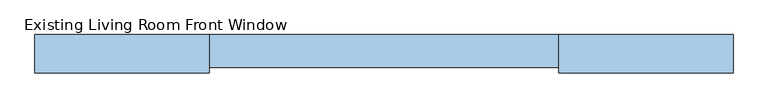
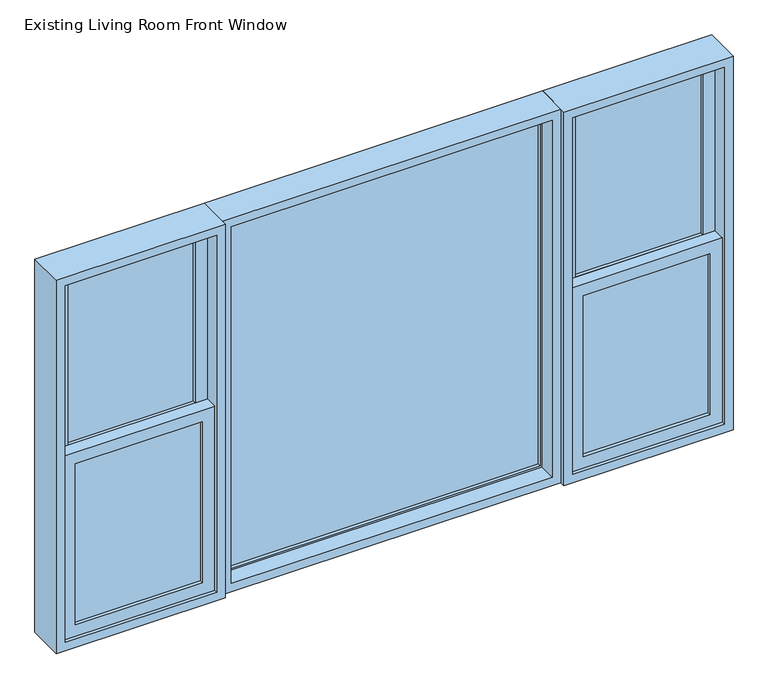
"""IFC4 building model written with IfcOpenShell, lengths in millimetres: window geometry, Existing Living Room Front Window."""

import ifcopenshell
import ifcopenshell.guid

model = None  # the IFC model being written
_history = None  # IfcOwnerHistory: only IFC2X3 demands one
_inside = {}  # id of a spatial element -> (the spatial element, [elements in it])
_under = {}  # id of a project, library or spatial element -> (it, [spatial elements below it])
_declared = {}  # id of a project -> (the project, [libraries it declares])
_typed = {}  # id of a type object -> (the type object, [elements of that type])
_made_of = {}  # id of a material, layer set ... -> (it, [elements and type objects made of it])


def new_model(schema):
    """Start an empty IFC model of exactly this schema.

    Asked for "IFC4X3", IfcOpenShell would pick the latest addendum, in which some entities
    have other attributes; the version numbers below select the first issue.
    IFC2X3 requires an IfcOwnerHistory on every rooted entity: one is made here for all.
    """
    global model, _history
    if schema == "IFC4X3":
        model = ifcopenshell.file(schema_version=(4, 3, 0, 0))
    else:
        model = ifcopenshell.file(schema=schema)
    _inside.clear()
    _under.clear()
    _declared.clear()
    _typed.clear()
    _made_of.clear()
    _history = None
    if model.schema == "IFC2X3":
        org = make("IfcOrganization", Name="unknown")
        user = make(
            "IfcPersonAndOrganization",
            ThePerson=make("IfcPerson", FamilyName="unknown"),
            TheOrganization=org,
        )
        app = make(
            "IfcApplication",
            ApplicationDeveloper=org,
            Version="unknown",
            ApplicationFullName="unknown",
            ApplicationIdentifier="unknown",
        )
        _history = make(
            "IfcOwnerHistory",
            OwningUser=user,
            OwningApplication=app,
            ChangeAction="ADDED",
            CreationDate=0,
        )
    return model


def make(cls, **values):
    """One entity of the class cls with the attributes given. An attribute that is None is left unset."""
    return model.create_entity(
        cls, **{name: value for name, value in values.items() if value is not None}
    )


def rooted(cls, **values):
    """An entity with a GlobalId (a new one), such as an element, a storey or a relation."""
    return make(cls, GlobalId=ifcopenshell.guid.new(), OwnerHistory=_history, **values)


def si_unit(unit_type, name, prefix=None):
    """IfcSIUnit, for example si_unit("LENGTHUNIT", "METRE", prefix="MILLI")."""
    return make("IfcSIUnit", UnitType=unit_type, Prefix=prefix, Name=name)


def assignment(units):
    """IfcUnitAssignment: the units of a project."""
    return None if units is None else make("IfcUnitAssignment", Units=units)


def point(xyz):
    """IfcCartesianPoint."""
    return None if xyz is None else make("IfcCartesianPoint", Coordinates=xyz)


def direction(xyz):
    """IfcDirection."""
    return None if xyz is None else make("IfcDirection", DirectionRatios=xyz)


def frame(location, z_axis=None, x_axis=None):
    """IfcAxis2Placement3D, a coordinate frame: its origin and axes. An axis left out is left unset."""
    return make(
        "IfcAxis2Placement3D",
        Location=point(location),
        Axis=direction(z_axis),
        RefDirection=direction(x_axis),
    )


def origin():
    """The frame at (0, 0, 0) with its axes left unset."""
    return frame((0.0, 0.0, 0.0))


def place(relative_to, where):
    """IfcLocalPlacement: puts the frame where relative to a parent placement (None: the world)."""
    return make(
        "IfcLocalPlacement", PlacementRelTo=relative_to, RelativePlacement=where
    )


def context(
    kind, dimensions, precision=None, world=None, true_north=None, identifier=None
):
    """IfcGeometricRepresentationContext, for example the 3D "Model" context."""
    return make(
        "IfcGeometricRepresentationContext",
        ContextIdentifier=identifier,
        ContextType=kind,
        CoordinateSpaceDimension=dimensions,
        Precision=precision,
        WorldCoordinateSystem=world,
        TrueNorth=true_north,
    )


def project(units=None, contexts=None):
    """IfcProject with its units and contexts."""
    return rooted(
        "IfcProject",
        Name="project",
        RepresentationContexts=contexts,
        UnitsInContext=assignment(units),
    )


def spatial(cls, under=None, at=None, **own):
    """A site, building, storey or space (cls), placed at a placement, below another one or the project."""
    s = rooted(cls, ObjectPlacement=at, **own)
    if under is not None:
        _under.setdefault(under.id(), (under, []))[1].append(s)
    return s


def polyline(points):
    """IfcPolyline through the points."""
    return make("IfcPolyline", Points=[point(p) for p in points])


def outline(outer, holes=None, kind="AREA"):
    """IfcArbitraryClosedProfileDef: a profile drawn as a closed curve; with holes, ...WithVoids."""
    if holes is None:
        return make("IfcArbitraryClosedProfileDef", ProfileType=kind, OuterCurve=outer)
    return make(
        "IfcArbitraryProfileDefWithVoids",
        ProfileType=kind,
        OuterCurve=outer,
        InnerCurves=holes,
    )


def extrude(swept, where, along, depth):
    """IfcExtrudedAreaSolid: the profile swept, set in the frame where, extruded along a direction by depth."""
    return make(
        "IfcExtrudedAreaSolid",
        SweptArea=swept,
        Position=where,
        ExtrudedDirection=direction(along),
        Depth=depth,
    )


def faces_of(points, faces, orient=None, outer=None):
    """IfcFace entities. A face is a list of loops; a loop is a list of indices into points, from 0.

    orient and outer hold one flag for each loop. By default every Orientation is true, the
    first loop of a face is its IfcFaceOuterBound and the others are IfcFaceBound.
    """
    made = []
    for i, loops in enumerate(faces):
        bounds = []
        for j, loop in enumerate(loops):
            is_outer = j == 0 if outer is None else outer[i][j]
            bounds.append(
                make(
                    "IfcFaceOuterBound" if is_outer else "IfcFaceBound",
                    Bound=make("IfcPolyLoop", Polygon=[points[k] for k in loop]),
                    Orientation=True if orient is None else orient[i][j],
                )
            )
        made.append(make("IfcFace", Bounds=bounds))
    return made


def faceted_brep(points, faces, orient=None, outer=None, voids=None):
    """IfcFacetedBrep: a solid bounded by flat faces; with voids (closed shells), ...WithVoids."""
    shared = [point(p) for p in points]
    hull = make("IfcClosedShell", CfsFaces=faces_of(shared, faces, orient, outer))
    if voids is None:
        return make("IfcFacetedBrep", Outer=hull)
    return make(
        "IfcFacetedBrepWithVoids",
        Outer=hull,
        Voids=[
            make(cls, CfsFaces=faces_of(shared, fs, o, b)) for cls, fs, o, b in voids
        ],
    )


def shape(context_of_items, identifier, shape_type, items):
    """IfcShapeRepresentation: the items that make up one representation, for example the "Body"."""
    return make(
        "IfcShapeRepresentation",
        ContextOfItems=context_of_items,
        RepresentationIdentifier=identifier,
        RepresentationType=shape_type,
        Items=items,
    )


def source(mapping_origin, context_of_items, identifier, shape_type, items):
    """IfcRepresentationMap: a shape defined once, which mapped items show again and again."""
    return make(
        "IfcRepresentationMap",
        MappingOrigin=mapping_origin,
        MappedRepresentation=shape(context_of_items, identifier, shape_type, items),
    )


def transform(
    local_origin,
    x_axis=None,
    y_axis=None,
    z_axis=None,
    scale=None,
    scale2=None,
    scale3=None,
    uniform=True,
):
    """IfcCartesianTransformationOperator3D, or its non-uniform kind. x_axis, y_axis, z_axis: its Axis1, 2, 3."""
    if uniform:
        return make(
            "IfcCartesianTransformationOperator3D",
            Axis1=direction(x_axis),
            Axis2=direction(y_axis),
            LocalOrigin=point(local_origin),
            Scale=scale,
            Axis3=direction(z_axis),
        )
    return make(
        "IfcCartesianTransformationOperator3DnonUniform",
        Axis1=direction(x_axis),
        Axis2=direction(y_axis),
        LocalOrigin=point(local_origin),
        Scale=scale,
        Axis3=direction(z_axis),
        Scale2=scale2,
        Scale3=scale3,
    )


def mapped(mapping_source, mapping_target):
    """IfcMappedItem: shows the shape of a source again, moved by a transform."""
    return make(
        "IfcMappedItem", MappingSource=mapping_source, MappingTarget=mapping_target
    )


def made_of(thing, what):
    """Note that an element or type object is made of a material, layer set ...; save() writes the relation."""
    if what is not None:
        _made_of.setdefault(what.id(), (what, []))[1].append(thing)
    return thing


def element(
    cls,
    number,
    at=None,
    inside=None,
    cuts=None,
    type_object=None,
    material=None,
    context=None,
    identifier="Body",
    shape_type=None,
    held_by="IfcProductDefinitionShape",
    body=None,
    shapes=None,
    **own,
):
    """One element of the class cls, such as IfcWall. Its Tag is "e" and its number.

    at: its placement. inside: the storey or other place that contains it. cuts: it is an
    opening in that element (IfcRelVoidsElement). A single representation is given by context,
    identifier, shape_type and body (its items); several are given by shapes. held_by: the class
    of the entity that holds the representations. save() writes the other relations.
    """
    e = rooted(cls, Tag="e%d" % number, ObjectPlacement=at, **own)
    if body is not None:
        shapes = [shape(context, identifier, shape_type, body)]
    if shapes is not None:
        e.Representation = make(held_by, Representations=shapes)
    if inside is not None:
        _inside.setdefault(inside.id(), (inside, []))[1].append(e)
    if cuts is not None:
        rooted(
            "IfcRelVoidsElement", RelatingBuildingElement=cuts, RelatedOpeningElement=e
        )
    if type_object is not None:
        _typed.setdefault(type_object.id(), (type_object, []))[1].append(e)
    return made_of(e, material)


def aggregate(whole, parts):
    """IfcRelAggregates: a whole, such as a stair, and the parts it consists of."""
    return rooted("IfcRelAggregates", RelatingObject=whole, RelatedObjects=parts)


def save(model, path):
    """Write the relations noted so far, then the file.

    IfcRelAggregates (storeys below a building ...), IfcRelContainedInSpatialStructure (elements
    in a storey), IfcRelDefinesByType, IfcRelAssociatesMaterial and IfcRelDeclares: one each for
    every whole, place, type object, material and project.
    """
    for whole, parts in _under.values():
        aggregate(whole, parts)
    for where, things in _inside.values():
        rooted(
            "IfcRelContainedInSpatialStructure",
            RelatedElements=things,
            RelatingStructure=where,
        )
    for kind, things in _typed.values():
        rooted("IfcRelDefinesByType", RelatedObjects=things, RelatingType=kind)
    for what, things in _made_of.values():
        rooted("IfcRelAssociatesMaterial", RelatedObjects=things, RelatingMaterial=what)
    for by, libraries in _declared.values():
        rooted("IfcRelDeclares", RelatingContext=by, RelatedDefinitions=libraries)
    model.write(path)


def existing_living_room_front_window_f3d2da23(model_context):
    return source(origin(), model_context, "Body", "SolidModel", [
        extrude(outline(polyline([(-1143.0, 82.55), (-685.8, 82.55), (-685.8, 76.2), (-1143.0, 76.2), (-1143.0, 82.55)])), frame((0.0, 0.0, 990.6), z_axis=(0.0, 0.0, 1.0), x_axis=(1.0, 0.0, 0.0)), (0.0, 0.0, 1.0), 612.775),
        extrude(outline(polyline([(-685.8, 69.85), (-685.8, 63.5), (-1143.0, 63.5), (-1143.0, 69.85), (-685.8, 69.85)])), frame((0.0, 0.0, 990.6), z_axis=(0.0, 0.0, 1.0), x_axis=(1.0, 0.0, 0.0)), (0.0, 0.0, 1.0), 612.775),
        extrude(outline(polyline([(-1143.0, 127.0), (-685.8, 127.0), (-685.8, 120.65), (-1143.0, 120.65), (-1143.0, 127.0)])), frame((0.0, 0.0, 1647.825), z_axis=(0.0, 0.0, 1.0), x_axis=(1.0, 0.0, 0.0)), (0.0, 0.0, 1.0), 612.775),
        extrude(outline(polyline([(-685.8, 114.3), (-685.8, 107.95), (-1143.0, 107.95), (-1143.0, 114.3), (-685.8, 114.3)])), frame((0.0, 0.0, 1647.825), z_axis=(0.0, 0.0, 1.0), x_axis=(1.0, 0.0, 0.0)), (0.0, 0.0, 1.0), 612.775),
        extrude(outline(polyline([(1647.825, -641.35), (1647.825, -1187.45), (946.15, -1187.45), (946.15, -641.35), (1647.825, -641.35)]), holes=[polyline([(1603.375, -1143.0), (1603.375, -685.8), (990.6, -685.8), (990.6, -1143.0), (1603.375, -1143.0)])]), frame((0.0, 50.8, 0.0), z_axis=(0.0, 1.0, 0.0), x_axis=(0.0, 0.0, 1.0)), (0.0, 0.0, 1.0), 44.45),
        extrude(outline(polyline([(2305.05, -641.35), (2305.05, -1187.45), (1603.375, -1187.45), (1603.375, -641.35), (2305.05, -641.35)]), holes=[polyline([(2260.6, -1143.0), (2260.6, -685.8), (1647.825, -685.8), (1647.825, -1143.0), (2260.6, -1143.0)])]), frame((0.0, 95.25, 0.0), z_axis=(0.0, 1.0, 0.0), x_axis=(0.0, 0.0, 1.0)), (0.0, 0.0, 1.0), 44.45),
        extrude(outline(polyline([(2336.8, -609.6), (2336.8, -1219.2), (914.4, -1219.2), (914.4, -609.6), (2336.8, -609.6)]), holes=[polyline([(2305.05, -1187.45), (2305.05, -641.35), (946.15, -641.35), (946.15, -1187.45), (2305.05, -1187.45)])]), frame((0.0, 38.1, 0.0), z_axis=(0.0, 1.0, 0.0), x_axis=(0.0, 0.0, 1.0)), (0.0, 0.0, 1.0), 133.35),
        extrude(outline(polyline([(685.8, 82.55), (1143.0, 82.55), (1143.0, 76.2), (685.8, 76.2), (685.8, 82.55)])), frame((0.0, 0.0, 990.6), z_axis=(0.0, 0.0, 1.0), x_axis=(1.0, 0.0, 0.0)), (0.0, 0.0, 1.0), 612.775),
        extrude(outline(polyline([(1143.0, 69.85), (1143.0, 63.5), (685.8, 63.5), (685.8, 69.85), (1143.0, 69.85)])), frame((0.0, 0.0, 990.6), z_axis=(0.0, 0.0, 1.0), x_axis=(1.0, 0.0, 0.0)), (0.0, 0.0, 1.0), 612.775),
        extrude(outline(polyline([(685.8, 127.0), (1143.0, 127.0), (1143.0, 120.65), (685.8, 120.65), (685.8, 127.0)])), frame((0.0, 0.0, 1647.825), z_axis=(0.0, 0.0, 1.0), x_axis=(1.0, 0.0, 0.0)), (0.0, 0.0, 1.0), 612.775),
        extrude(outline(polyline([(1143.0, 114.3), (1143.0, 107.95), (685.8, 107.95), (685.8, 114.3), (1143.0, 114.3)])), frame((0.0, 0.0, 1647.825), z_axis=(0.0, 0.0, 1.0), x_axis=(1.0, 0.0, 0.0)), (0.0, 0.0, 1.0), 612.775),
        extrude(outline(polyline([(1647.825, 1187.45), (1647.825, 641.35), (946.15, 641.35), (946.15, 1187.45), (1647.825, 1187.45)]), holes=[polyline([(1603.375, 685.8), (1603.375, 1143.0), (990.6, 1143.0), (990.6, 685.8), (1603.375, 685.8)])]), frame((0.0, 50.8, 0.0), z_axis=(0.0, 1.0, 0.0), x_axis=(0.0, 0.0, 1.0)), (0.0, 0.0, 1.0), 44.45),
        extrude(outline(polyline([(2305.05, 1187.45), (2305.05, 641.35), (1603.375, 641.35), (1603.375, 1187.45), (2305.05, 1187.45)]), holes=[polyline([(2260.6, 685.8), (2260.6, 1143.0), (1647.825, 1143.0), (1647.825, 685.8), (2260.6, 685.8)])]), frame((0.0, 95.25, 0.0), z_axis=(0.0, 1.0, 0.0), x_axis=(0.0, 0.0, 1.0)), (0.0, 0.0, 1.0), 44.45),
        extrude(outline(polyline([(2336.8, 1219.2), (2336.8, 609.6), (914.4, 609.6), (914.4, 1219.2), (2336.8, 1219.2)]), holes=[polyline([(2305.05, 641.35), (2305.05, 1187.45), (946.15, 1187.45), (946.15, 641.35), (2305.05, 641.35)])]), frame((0.0, 38.1, 0.0), z_axis=(0.0, 1.0, 0.0), x_axis=(0.0, 0.0, 1.0)), (0.0, 0.0, 1.0), 133.35),
        extrude(outline(polyline([(-571.5, 152.4), (571.5, 152.4), (571.5, 146.05), (-571.5, 146.05), (-571.5, 152.4)])), frame((0.0, 0.0, 952.5), z_axis=(0.0, 0.0, 1.0), x_axis=(1.0, 0.0, 0.0)), (0.0, 0.0, 1.0), 1346.2),
        extrude(outline(polyline([(571.5, 133.35), (-571.5, 133.35), (-571.5, 139.7), (571.5, 139.7), (571.5, 133.35)])), frame((0.0, 0.0, 952.5), z_axis=(0.0, 0.0, 1.0), x_axis=(1.0, 0.0, 0.0)), (0.0, 0.0, 1.0), 1346.2),
        extrude(outline(polyline([(927.1, -596.9), (927.1, 596.9), (2324.1, 596.9), (2324.1, -596.9), (927.1, -596.9)]), holes=[polyline([(952.5, 571.5), (952.5, -571.5), (2298.7, -571.5), (2298.7, 571.5), (952.5, 571.5)])]), frame((0.0, 120.65, 0.0), z_axis=(0.0, 1.0, 0.0), x_axis=(0.0, 0.0, 1.0)), (0.0, 0.0, 1.0), 44.45),
        faceted_brep([(-609.6, 57.15, 2336.8), (609.6, 57.15, 2336.8), (609.6, 171.45, 2336.8), (-609.6, 171.45, 2336.8), (609.6, 57.15, 914.4), (609.6, 171.45, 914.4), (-609.6, 57.15, 914.4), (-609.6, 171.45, 914.4), (-577.85, 57.15, 2305.05), (577.85, 57.15, 2305.05), (577.85, 57.15, 946.15), (-577.85, 57.15, 946.15), (596.9, 171.45, 2324.1), (-596.9, 171.45, 2324.1), (-596.9, 171.45, 927.1), (596.9, 171.45, 927.1), (-577.85, 120.65, 2305.05), (577.85, 120.65, 2305.05), (596.9, 120.65, 2324.1), (-596.9, 120.65, 2324.1), (577.85, 120.65, 946.15), (596.9, 120.65, 927.1), (-577.85, 120.65, 946.15), (-596.9, 120.65, 927.1)], [[[0, 1, 2, 3]], [[1, 4, 5, 2]], [[4, 6, 7, 5]], [[1, 0, 6, 4], [8, 9, 10, 11]], [[6, 0, 3, 7]], [[3, 2, 5, 7], [12, 13, 14, 15]], [[16, 17, 9, 8]], [[13, 12, 18, 19]], [[17, 20, 10, 9]], [[12, 15, 21, 18]], [[20, 22, 11, 10]], [[15, 14, 23, 21]], [[22, 16, 8, 11]], [[19, 18, 21, 23], [17, 16, 22, 20]], [[14, 13, 19, 23]]]),
    ])


if __name__ == "__main__":
    model = new_model("IFC4")
    model_context = context("Model", 3, world=origin())
    ifc_project = project(units=[si_unit("LENGTHUNIT", "METRE", prefix="MILLI")], contexts=[model_context])
    site = spatial("IfcSite", under=ifc_project)
    building = spatial("IfcBuilding", under=site)
    placement = place(None, origin())
    existing_living_room_front_window_shape = existing_living_room_front_window_f3d2da23(model_context)
    element("IfcWindow", 1, ObjectType="Existing Living Room Front Window : (2) 2'-0\" x 4'-8\" DH + 4'-0\" x 4'-8\" FX", at=placement, inside=building, context=model_context, shape_type="MappedRepresentation", body=[
        mapped(existing_living_room_front_window_shape, transform((0.0, 0.0, 0.0), x_axis=(1.0, 0.0, 0.0), y_axis=(0.0, 1.0, 0.0), z_axis=(0.0, 0.0, 1.0))),
    ])
    save(model, "model.ifc")

# Revit data of these elements
# Type "Existing Living Room Front Window : (2) 2'-0\" x 4'-8\" DH + 4'-0\" x 4'-8\" FX"
#   Type Mark = "21"
#   Window Inset = 0' - 0 3/4"
#   Side Window Width = 2' - 0"
#   Side Window Location = 2' - 0"
#   Middle Window Width = 4' - 0"
#   Height = 4' - 8"
#   Default Sill Height = 3' - 0"
#   Width = 8' - 0"
#   Top Muntin Visibility = yes
#   Interior Trim Visibility [instance default] = yes
#   Fixed Muntin Visibility = no
#   Exterior Trim Visibility [instance default] = yes
#   Bottom Muntin Visibility = yes
#   Sash Material = Sash
#   Interior Trim = Trim-Window-Interior-Flat : Picture Frame
#   Interior Trim Material = Wood - Stained
#   Interior Frame Material = Wood - Stained
#   Glass Pane Material = Glass
#   Exterior Trim Material = Clad - White
#   Exterior Trim = Trim-Window-Exterior-Flat : with Sill
#   Exterior Frame Material = Clad - White
#   Rough Width = 0
#   Rough Height = 0
#   Wall Closure = (empty or 0)
# Element 1 (IfcWindow, "Existing Living Room Front Window : (2) 2'-0\" x 4'-8\" DH + 4'-0\" x 4'-8\" FX")
#   Materials on its faces: "Wood - Stained", "Glass", "Clad - White"
# Materials
#   "Sash": class "Wood", colour RGB 224 178 126, transparency 0, Cost = 0
#   "Wood - Stained": class "Wood", colour RGB 224 178 126, transparency 0, Cost = 0
#   "Glass": class "Glass", colour RGB 0 128 192, transparency 0.75, Description = "Soda Lime Glass", Cost = 0
#   "Clad - White": class "Wood", colour RGB 242 242 238, transparency 0, Cost = 0
